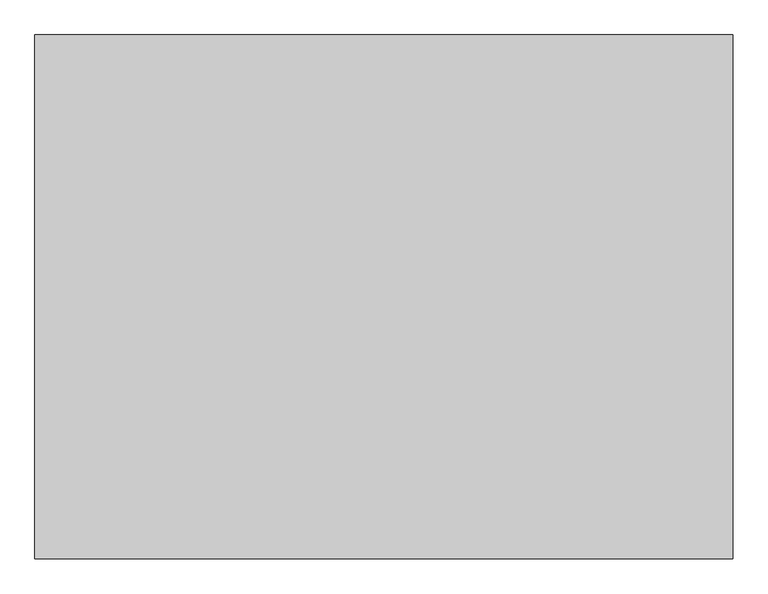
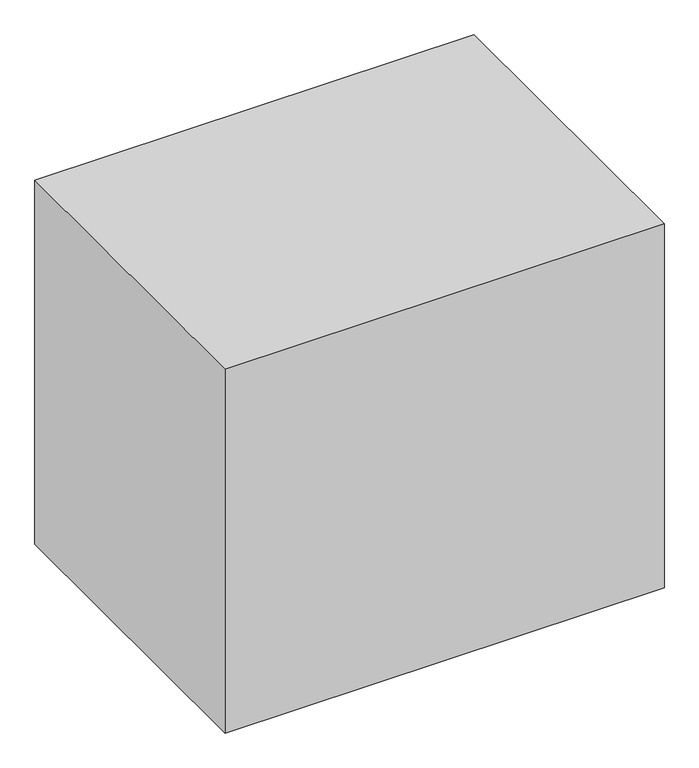
"""IFC4 building model written with IfcOpenShell, lengths in millimetres: proxy geometry, Space Planning Box_hec : Space Planning Box_hec."""

import ifcopenshell
import ifcopenshell.guid

model = None  # the IFC model being written
_history = None  # IfcOwnerHistory: only IFC2X3 demands one
_inside = {}  # id of a spatial element -> (the spatial element, [elements in it])
_under = {}  # id of a project, library or spatial element -> (it, [spatial elements below it])
_declared = {}  # id of a project -> (the project, [libraries it declares])
_typed = {}  # id of a type object -> (the type object, [elements of that type])
_made_of = {}  # id of a material, layer set ... -> (it, [elements and type objects made of it])


def new_model(schema):
    """Start an empty IFC model of exactly this schema.

    Asked for "IFC4X3", IfcOpenShell would pick the latest addendum, in which some entities
    have other attributes; the version numbers below select the first issue.
    IFC2X3 requires an IfcOwnerHistory on every rooted entity: one is made here for all.
    """
    global model, _history
    if schema == "IFC4X3":
        model = ifcopenshell.file(schema_version=(4, 3, 0, 0))
    else:
        model = ifcopenshell.file(schema=schema)
    _inside.clear()
    _under.clear()
    _declared.clear()
    _typed.clear()
    _made_of.clear()
    _history = None
    if model.schema == "IFC2X3":
        org = make("IfcOrganization", Name="unknown")
        user = make(
            "IfcPersonAndOrganization",
            ThePerson=make("IfcPerson", FamilyName="unknown"),
            TheOrganization=org,
        )
        app = make(
            "IfcApplication",
            ApplicationDeveloper=org,
            Version="unknown",
            ApplicationFullName="unknown",
            ApplicationIdentifier="unknown",
        )
        _history = make(
            "IfcOwnerHistory",
            OwningUser=user,
            OwningApplication=app,
            ChangeAction="ADDED",
            CreationDate=0,
        )
    return model


def make(cls, **values):
    """One entity of the class cls with the attributes given. An attribute that is None is left unset."""
    return model.create_entity(
        cls, **{name: value for name, value in values.items() if value is not None}
    )


def rooted(cls, **values):
    """An entity with a GlobalId (a new one), such as an element, a storey or a relation."""
    return make(cls, GlobalId=ifcopenshell.guid.new(), OwnerHistory=_history, **values)


def si_unit(unit_type, name, prefix=None):
    """IfcSIUnit, for example si_unit("LENGTHUNIT", "METRE", prefix="MILLI")."""
    return make("IfcSIUnit", UnitType=unit_type, Prefix=prefix, Name=name)


def assignment(units):
    """IfcUnitAssignment: the units of a project."""
    return None if units is None else make("IfcUnitAssignment", Units=units)


def point(xyz):
    """IfcCartesianPoint."""
    return None if xyz is None else make("IfcCartesianPoint", Coordinates=xyz)


def direction(xyz):
    """IfcDirection."""
    return None if xyz is None else make("IfcDirection", DirectionRatios=xyz)


def frame(location, z_axis=None, x_axis=None):
    """IfcAxis2Placement3D, a coordinate frame: its origin and axes. An axis left out is left unset."""
    return make(
        "IfcAxis2Placement3D",
        Location=point(location),
        Axis=direction(z_axis),
        RefDirection=direction(x_axis),
    )


def origin():
    """The frame at (0, 0, 0) with its axes left unset."""
    return frame((0.0, 0.0, 0.0))


def origin_with_axes():
    """The frame at (0, 0, 0) with the z axis (0, 0, 1) and the x axis (1, 0, 0) written out."""
    return frame((0.0, 0.0, 0.0), z_axis=(0.0, 0.0, 1.0), x_axis=(1.0, 0.0, 0.0))


def place(relative_to, where):
    """IfcLocalPlacement: puts the frame where relative to a parent placement (None: the world)."""
    return make(
        "IfcLocalPlacement", PlacementRelTo=relative_to, RelativePlacement=where
    )


def context(
    kind, dimensions, precision=None, world=None, true_north=None, identifier=None
):
    """IfcGeometricRepresentationContext, for example the 3D "Model" context."""
    return make(
        "IfcGeometricRepresentationContext",
        ContextIdentifier=identifier,
        ContextType=kind,
        CoordinateSpaceDimension=dimensions,
        Precision=precision,
        WorldCoordinateSystem=world,
        TrueNorth=true_north,
    )


def project(units=None, contexts=None):
    """IfcProject with its units and contexts."""
    return rooted(
        "IfcProject",
        Name="project",
        RepresentationContexts=contexts,
        UnitsInContext=assignment(units),
    )


def spatial(cls, under=None, at=None, **own):
    """A site, building, storey or space (cls), placed at a placement, below another one or the project."""
    s = rooted(cls, ObjectPlacement=at, **own)
    if under is not None:
        _under.setdefault(under.id(), (under, []))[1].append(s)
    return s


def polyline(points):
    """IfcPolyline through the points."""
    return make("IfcPolyline", Points=[point(p) for p in points])


def outline(outer, holes=None, kind="AREA"):
    """IfcArbitraryClosedProfileDef: a profile drawn as a closed curve; with holes, ...WithVoids."""
    if holes is None:
        return make("IfcArbitraryClosedProfileDef", ProfileType=kind, OuterCurve=outer)
    return make(
        "IfcArbitraryProfileDefWithVoids",
        ProfileType=kind,
        OuterCurve=outer,
        InnerCurves=holes,
    )


def extrude(swept, where, along, depth):
    """IfcExtrudedAreaSolid: the profile swept, set in the frame where, extruded along a direction by depth."""
    return make(
        "IfcExtrudedAreaSolid",
        SweptArea=swept,
        Position=where,
        ExtrudedDirection=direction(along),
        Depth=depth,
    )


def shape(context_of_items, identifier, shape_type, items):
    """IfcShapeRepresentation: the items that make up one representation, for example the "Body"."""
    return make(
        "IfcShapeRepresentation",
        ContextOfItems=context_of_items,
        RepresentationIdentifier=identifier,
        RepresentationType=shape_type,
        Items=items,
    )


def source(mapping_origin, context_of_items, identifier, shape_type, items):
    """IfcRepresentationMap: a shape defined once, which mapped items show again and again."""
    return make(
        "IfcRepresentationMap",
        MappingOrigin=mapping_origin,
        MappedRepresentation=shape(context_of_items, identifier, shape_type, items),
    )


def transform(
    local_origin,
    x_axis=None,
    y_axis=None,
    z_axis=None,
    scale=None,
    scale2=None,
    scale3=None,
    uniform=True,
):
    """IfcCartesianTransformationOperator3D, or its non-uniform kind. x_axis, y_axis, z_axis: its Axis1, 2, 3."""
    if uniform:
        return make(
            "IfcCartesianTransformationOperator3D",
            Axis1=direction(x_axis),
            Axis2=direction(y_axis),
            LocalOrigin=point(local_origin),
            Scale=scale,
            Axis3=direction(z_axis),
        )
    return make(
        "IfcCartesianTransformationOperator3DnonUniform",
        Axis1=direction(x_axis),
        Axis2=direction(y_axis),
        LocalOrigin=point(local_origin),
        Scale=scale,
        Axis3=direction(z_axis),
        Scale2=scale2,
        Scale3=scale3,
    )


def mapped(mapping_source, mapping_target):
    """IfcMappedItem: shows the shape of a source again, moved by a transform."""
    return make(
        "IfcMappedItem", MappingSource=mapping_source, MappingTarget=mapping_target
    )


def made_of(thing, what):
    """Note that an element or type object is made of a material, layer set ...; save() writes the relation."""
    if what is not None:
        _made_of.setdefault(what.id(), (what, []))[1].append(thing)
    return thing


def element(
    cls,
    number,
    at=None,
    inside=None,
    cuts=None,
    type_object=None,
    material=None,
    context=None,
    identifier="Body",
    shape_type=None,
    held_by="IfcProductDefinitionShape",
    body=None,
    shapes=None,
    **own,
):
    """One element of the class cls, such as IfcWall. Its Tag is "e" and its number.

    at: its placement. inside: the storey or other place that contains it. cuts: it is an
    opening in that element (IfcRelVoidsElement). A single representation is given by context,
    identifier, shape_type and body (its items); several are given by shapes. held_by: the class
    of the entity that holds the representations. save() writes the other relations.
    """
    e = rooted(cls, Tag="e%d" % number, ObjectPlacement=at, **own)
    if body is not None:
        shapes = [shape(context, identifier, shape_type, body)]
    if shapes is not None:
        e.Representation = make(held_by, Representations=shapes)
    if inside is not None:
        _inside.setdefault(inside.id(), (inside, []))[1].append(e)
    if cuts is not None:
        rooted(
            "IfcRelVoidsElement", RelatingBuildingElement=cuts, RelatedOpeningElement=e
        )
    if type_object is not None:
        _typed.setdefault(type_object.id(), (type_object, []))[1].append(e)
    return made_of(e, material)


def aggregate(whole, parts):
    """IfcRelAggregates: a whole, such as a stair, and the parts it consists of."""
    return rooted("IfcRelAggregates", RelatingObject=whole, RelatedObjects=parts)


def save(model, path):
    """Write the relations noted so far, then the file.

    IfcRelAggregates (storeys below a building ...), IfcRelContainedInSpatialStructure (elements
    in a storey), IfcRelDefinesByType, IfcRelAssociatesMaterial and IfcRelDeclares: one each for
    every whole, place, type object, material and project.
    """
    for whole, parts in _under.values():
        aggregate(whole, parts)
    for where, things in _inside.values():
        rooted(
            "IfcRelContainedInSpatialStructure",
            RelatedElements=things,
            RelatingStructure=where,
        )
    for kind, things in _typed.values():
        rooted("IfcRelDefinesByType", RelatedObjects=things, RelatingType=kind)
    for what, things in _made_of.values():
        rooted("IfcRelAssociatesMaterial", RelatedObjects=things, RelatingMaterial=what)
    for by, libraries in _declared.values():
        rooted("IfcRelDeclares", RelatingContext=by, RelatedDefinitions=libraries)
    model.write(path)


def generic_models_4c644d41(model_context):
    return source(origin(), model_context, "Body", "SweptSolid", [
        extrude(outline(polyline([(2000.0, 1500.0), (2000.0, -1500.0), (-2000.0, -1500.0), (-2000.0, 1500.0), (2000.0, 1500.0)])), origin_with_axes(), (0.0, 0.0, 1.0), 3500.0),
    ])


if __name__ == "__main__":
    model = new_model("IFC4")
    model_context = context("Model", 3, world=origin())
    ifc_project = project(units=[si_unit("LENGTHUNIT", "METRE", prefix="MILLI")], contexts=[model_context])
    site = spatial("IfcSite", under=ifc_project)
    building = spatial("IfcBuilding", under=site)
    placement = place(None, origin())
    generic_models_shape = generic_models_4c644d41(model_context)
    element("IfcBuildingElementProxy", 1, Name="Space Planning Box_hec : Space Planning Box_hec", ObjectType="Space Planning Box_hec : Space Planning Box_hec", at=placement, inside=building, context=model_context, shape_type="MappedRepresentation", body=[
        mapped(generic_models_shape, transform((0.0, 0.0, 0.0), x_axis=(1.0, 0.0, 0.0), y_axis=(0.0, 1.0, 0.0), z_axis=(0.0, 0.0, 1.0))),
    ])
    save(model, "model.ifc")

# Revit data of these elements
# Type "Space Planning Box_hec : Space Planning Box_hec"
#   Type Comments = "..."
#   Room Name [instance default] = "?"
#   Interior Finish [instance default] = ""
#   Exterior Finish [instance default] = ""
#   Department [instance default] = ""
#   Assembly Code = "..."
#   Width [instance default] = 1524 mm
#   Program Area [instance default] = 0.00 m²
#   Length [instance default] = 1524 mm
#   Height [instance default] = 1524 mm
#   Area [instance default] = 2.32258 m²
#   Fill Color [instance default] = Cyan
#   Default Elevation = 0
# Element 1 (IfcBuildingElementProxy, "Space Planning Box_hec : Space Planning Box_hec")
#   Room Name = "Elevator"
#   Department = "AR"
#   Width = 4000 mm
#   Length = 3000 mm
#   Height = 3500 mm
#   Area = 12.00 m²
#   Materials on its faces: "Cyan"
# Materials
#   "Cyan": class "Generic", colour RGB 0 255 255, transparency 0.2, Cost = 0
